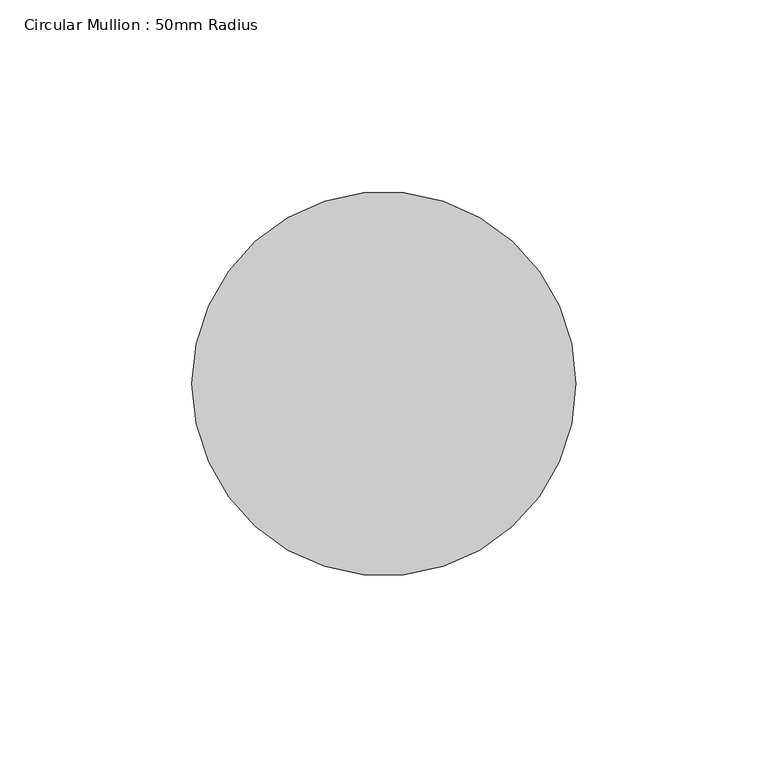
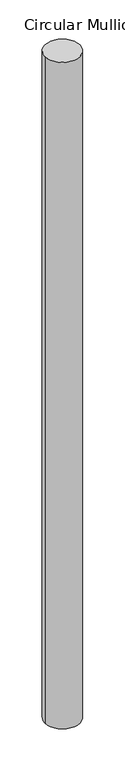
"""IFC4 building model written with IfcOpenShell, lengths in millimetres: member geometry, Circular Mullion : 50mm Radius."""

from ifc_helpers import new_model, si_unit, point, frame, frame_2d, origin, place, context, project, spatial, circle_curve, trimmed, segment, composite_curve, outline, extrude, source, transform, mapped, element, save


def circular_mullion_50mm_radius_c766e87e(model_context):
    return source(origin(), model_context, "Body", "SweptSolid", [
        extrude(outline(composite_curve([segment(trimmed(circle_curve(frame_2d((-50.0, 0.0)), 50.0), [point((0.0, 0.0))], [point((-100.0, 0.0))], False, "CARTESIAN"), True, "CONTINUOUS"), segment(trimmed(circle_curve(frame_2d((-50.0, 0.0)), 50.0), [point((-100.0, 0.0))], [point((0.0, 0.0))], False, "CARTESIAN"), True, "CONTINUOUS")], self_intersect=False)), frame((0.0, 0.0, -2005.2560832), z_axis=(0.0, 0.0, 1.0), x_axis=(1.0, 0.0, 0.0)), (0.0, 0.0, 1.0), 2005.2560832),
    ])


if __name__ == "__main__":
    model = new_model("IFC4")
    model_context = context("Model", 3, world=origin())
    ifc_project = project(units=[si_unit("LENGTHUNIT", "METRE", prefix="MILLI")], contexts=[model_context])
    site = spatial("IfcSite", under=ifc_project)
    building = spatial("IfcBuilding", under=site)
    placement = place(None, origin())
    circular_mullion_50mm_radius_shape = circular_mullion_50mm_radius_c766e87e(model_context)
    element("IfcMember", 1, ObjectType="Circular Mullion : 50mm Radius", at=placement, inside=building, context=model_context, shape_type="MappedRepresentation", body=[
        mapped(circular_mullion_50mm_radius_shape, transform((0.0, 0.0, 0.0), x_axis=(1.0, 0.0, 0.0), y_axis=(0.0, 1.0, 0.0), z_axis=(0.0, 0.0, 1.0))),
    ])
    save(model, "model.ifc")

# Revit data of these elements
# Type "Circular Mullion : 50mm Radius"
#   built-in parameter 1007350 = 0.164042 (stored number, unit not read)
# Element 1 (IfcMember, "Circular Mullion : 50mm Radius")
#   Materials on its faces: "Aluminium"
# Materials
#   "Aluminium": class "Metal", colour RGB 247 247 247, transparency 0, Description = "Aluminium 6061", Cost = 0
